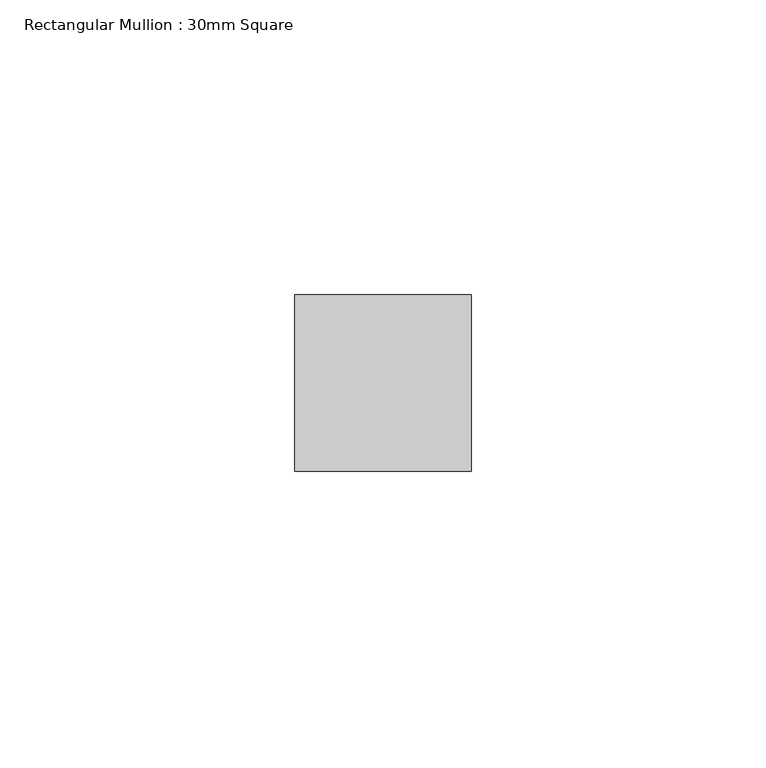
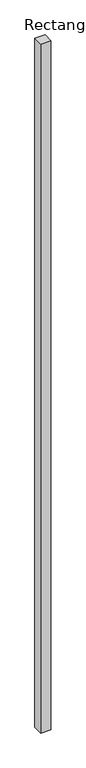
"""IFC4 building model written with IfcOpenShell, lengths in millimetres: member geometry, Rectangular Mullion : 30mm Square."""

from ifc_helpers import new_model, si_unit, frame, origin, place, context, project, spatial, polyline, outline, extrude, source, transform, mapped, element, save


def rectangular_mullion_30mm_square_fecaf73a(model_context):
    return source(origin(), model_context, "Body", "SweptSolid", [
        extrude(outline(polyline([(15.0, 15.0), (15.0, -15.0), (-15.0, -15.0), (-15.0, 15.0), (15.0, 15.0)])), frame((0.0, 0.0, -2152.3545613), z_axis=(0.0, 0.0, 1.0), x_axis=(1.0, 0.0, 0.0)), (0.0, 0.0, 1.0), 2152.3545613),
    ])


if __name__ == "__main__":
    model = new_model("IFC4")
    model_context = context("Model", 3, world=origin())
    ifc_project = project(units=[si_unit("LENGTHUNIT", "METRE", prefix="MILLI")], contexts=[model_context])
    site = spatial("IfcSite", under=ifc_project)
    building = spatial("IfcBuilding", under=site)
    placement = place(None, origin())
    rectangular_mullion_30mm_square_shape = rectangular_mullion_30mm_square_fecaf73a(model_context)
    element("IfcMember", 1, ObjectType="Rectangular Mullion : 30mm Square", at=placement, inside=building, context=model_context, shape_type="MappedRepresentation", body=[
        mapped(rectangular_mullion_30mm_square_shape, transform((0.0, 0.0, 0.0), x_axis=(1.0, 0.0, 0.0), y_axis=(0.0, 1.0, 0.0), z_axis=(0.0, 0.0, 1.0))),
    ])
    save(model, "model.ifc")

# Revit data of these elements
# Type "Rectangular Mullion : 30mm Square"
#   built-in parameter 1007304 = 0.0984252 (stored number, unit not read)
#   built-in parameter 1007301 = 0.0492126 (stored number, unit not read)
#   built-in parameter 1007300 = 0.0492126 (stored number, unit not read)
# Element 1 (IfcMember, "Rectangular Mullion : 30mm Square")
#   Materials on its faces: "Aluminum"
# Materials
#   "Aluminum": class "Metal", colour RGB 244 244 244, transparency 0, Description = "Aluminum 6061", Cost = 0
